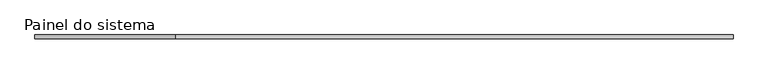
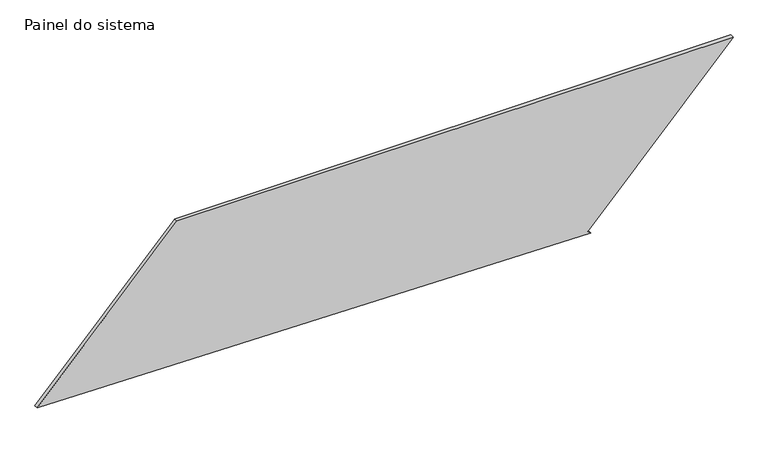
"""IFC4 building model written with IfcOpenShell, lengths in millimetres: plate geometry, Painel do sistema : Envidraçado."""

from ifc_helpers import new_model, si_unit, frame, origin, place, context, project, spatial, polyline, outline, extrude, source, transform, mapped, element, save


def painel_do_sistema_cdba6993(model_context):
    return source(origin(), model_context, "Body", "SweptSolid", [
        extrude(outline(polyline([(0.0, 1291.9713974), (17.1196584, 1273.7527998), (989.359926, 2187.3478881), (989.359926, -1308.5701498), (54.1719916, -2187.3478881), (0.0, 1291.9713974)])), frame((0.0, 24.5, 0.0), z_axis=(0.0, 1.0, 0.0), x_axis=(0.0, 0.0, 1.0)), (0.0, 0.0, 1.0), 25.0),
    ])


if __name__ == "__main__":
    model = new_model("IFC4")
    model_context = context("Model", 3, world=origin())
    ifc_project = project(units=[si_unit("LENGTHUNIT", "METRE", prefix="MILLI")], contexts=[model_context])
    site = spatial("IfcSite", under=ifc_project)
    building = spatial("IfcBuilding", under=site)
    placement = place(None, origin())
    painel_do_sistema_shape = painel_do_sistema_cdba6993(model_context)
    element("IfcPlate", 1, ObjectType="Painel do sistema : Envidraçado", at=placement, inside=building, context=model_context, shape_type="MappedRepresentation", body=[
        mapped(painel_do_sistema_shape, transform((0.0, 0.0, 0.0), x_axis=(1.0, 0.0, 0.0), y_axis=(0.0, 1.0, 0.0), z_axis=(0.0, 0.0, 1.0))),
    ])
    save(model, "model.ifc")

# Revit data of these elements
# Type "Painel do sistema : Envidraçado"
#   Construction Type Id = "GSP4R"
#   Analytic Construction = "Vidraça única Pilkington 1/8 pol"
#   Visual Light Transmittance = 0.9
#   Solar Heat Gain Coefficient = 0.86
#   Heat Transfer Coefficient (U) = 6.7069 W/(m²·K)
# Element 1 (IfcPlate, "Painel do sistema : Envidraçado")
#   Materials on its faces: "Vidro"
# Materials
#   "Vidro": class "Vidro", colour RGB 0 128 192, transparency 0.9, Description = "Vidro de sílica", Cost = 0
